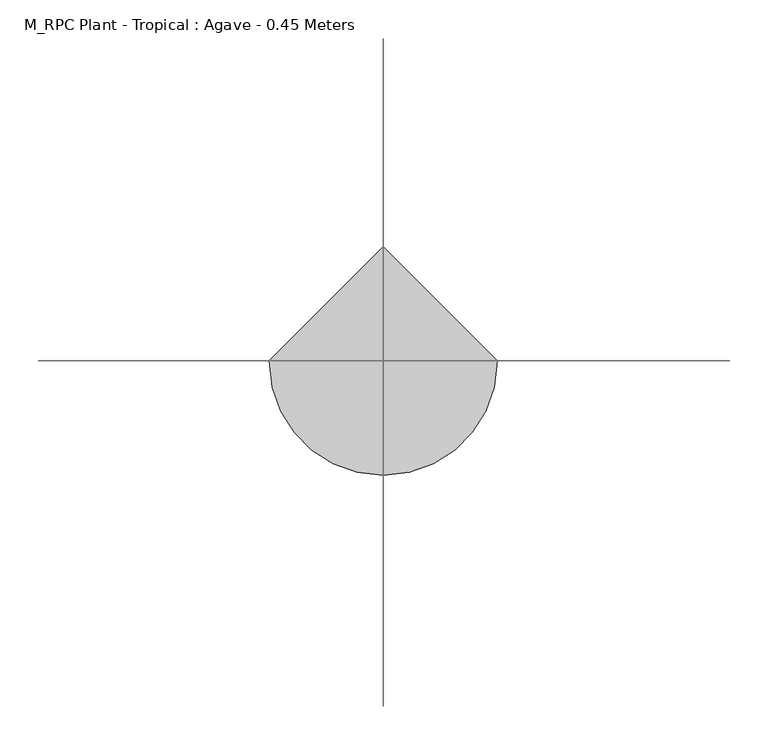
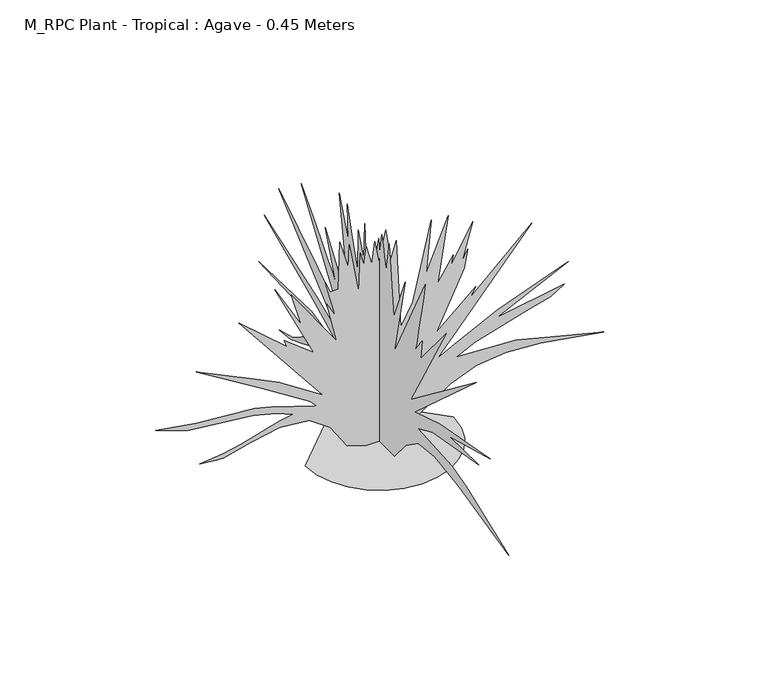
"""IFC4 building model written with IfcOpenShell, lengths in millimetres: geographic element geometry, M_RPC Plant - Tropical : Agave - 0.45 Meters."""

from ifc_helpers import new_model, si_unit, origin, place, context, project, spatial, triangles, source, transform, mapped, element, save


def m_rpc_plant_tropical_agave_0_45_meters_1685f993(model_context):
    return source(origin(), model_context, "Body", "Tessellation", [
        triangles([(-148.1386958, 0.0, 9.3e-06), (-144.2171964, -33.9885277, 9.3e-06), (-133.048683, -65.2018023, 9.3e-06), (-115.5276685, -92.7450748, 9.3e-06), (-92.5484025, -115.7243407, 9.3e-06), (-65.0051301, -133.2453552, 9.3e-06), (-33.7918577, -144.4138686, 9.3e-06), (0.1966776, -148.335368, 9.3e-06), (34.1851976, -144.4138686, 9.3e-06), (65.3984745, -133.2453552, 9.3e-06), (92.941747, -115.7243407, 9.3e-06), (115.921013, -92.7450748, 9.3e-06), (133.4420274, -65.2018023, 9.3e-06), (144.6105409, -33.9885277, 9.3e-06), (148.5320402, 1.3e-05, 9.3e-06), (0.1966516, 148.335368, 9.3e-06), (-24.3504259, 1.1e-06, 2.5e-06), (-64.1988793, 2e-06, 12.9348607), (-97.895905, 5e-07, 64.0713026), (-140.594189, 5e-07, 94.1593235), (-198.9417449, 2.8e-06, 99.5475847), (-255.4485429, 5.9e-06, 87.7748204), (-311.5910826, 9.2e-06, 73.8080584), (-324.2335885, 9.8e-06, 74.3145591), (-359.378609, 1.11e-05, 77.950311), (-313.1035629, 8.8e-06, 82.7858171), (-277.6960585, 6.8e-06, 90.344322), (-199.7057426, 2e-06, 113.0485956), (-172.7469775, 5e-07, 117.942592), (-204.8844963, 1.2e-06, 130.9928583), (-252.5285358, 2.5e-06, 143.4918682), (-382.9561306, 7.4e-06, 157.5558808), (-447.8461741, 8.9e-06, 179.7488939), (-367.8611217, 6.2e-06, 166.4181305), (-249.0960418, 1.6e-06, 156.7231191), (-216.6905162, 6e-07, 148.7013704), (-125.4831837, -1.6e-06, 119.1546001), (-138.0646922, -1.9e-06, 133.1736118), (-234.3990283, -1.3e-06, 193.9569111), (-366.6486231, -4e-07, 275.4877267), (-252.1085396, -2.1e-06, 220.5199336), (-200.6204942, -2.9e-06, 195.5036553), (-113.3644194, -3.3e-06, 138.5448591), (-281.816065, -8.5e-06, 349.4127929), (-184.8657327, -7.8e-06, 265.7927153), (-189.7134928, -8.4e-06, 280.3352324), (-131.5426884, -8.2e-06, 234.2839372), (-209.1037518, -1.44e-05, 395.4653234), (-155.7804623, -1.12e-05, 302.1502526), (-176.3827294, -1.45e-05, 372.4403117), (-85.4908937, -1.07e-05, 242.7671948), (-104.8811618, -1.49e-05, 327.6002798), (-87.9146465, -1.39e-05, 297.3027469), (-108.5169137, -1.76e-05, 374.8628019), (-97.9506527, -1.66e-05, 351.3077717), (-81.76514, -1.74e-05, 351.3277923), (-79.4313889, -2.33e-05, 450.0003668), (-62.2313804, -2.06e-05, 390.7203006), (-60.0411253, -2.35e-05, 437.880358), (-40.6511115, -1.79e-05, 330.02277), (-38.2271089, -2.29e-05, 412.4328197), (-30.9558549, -2.16e-05, 384.5578134), (-26.1083514, -2.4e-05, 422.1278312), (-15.2013409, -2.2e-05, 380.9228245), (-9.1419117, -2.5e-05, 426.9753551), (-0.6586671, -2.27e-05, 380.9228245), (12.6721065, -2.7e-05, 443.9403442), (23.5791135, -2.35e-05, 377.2877993), (34.4861967, -2.62e-05, 413.6428476), (42.9694566, -1.54e-05, 227.0126877), (67.2069761, -1.91e-05, 271.8527196), (104.0335027, -3.03e-05, 433.0253491), (93.8687435, -2.34e-05, 323.9627475), (138.4672839, -3.17e-05, 430.0728404), (116.8945182, -2.27e-05, 294.8777314), (148.4037959, -2.69e-05, 343.3552774), (143.5562902, -2.54e-05, 321.5402573), (187.184323, -3.2e-05, 400.312811), (165.3703021, -2.65e-05, 322.7527559), (177.4890573, -2.84e-05, 345.7777677), (170.9330439, -2.58e-05, 308.0802504), (114.4707654, -1.64e-05, 190.6558953), (193.2438187, -2.4e-05, 260.9452096), (181.1248092, -2.22e-05, 240.3434511), (305.9494211, -3.46e-05, 355.4727791), (116.8945182, -1.32e-05, 136.120861), (156.175787, -1.61e-05, 155.588123), (236.8716063, -2.2e-05, 195.5036553), (378.6619886, -3.14e-05, 248.8267087), (235.6598525, -2.1e-05, 179.7488939), (371.0494809, -2.83e-05, 203.1156725), (343.871961, -2.62e-05, 186.8916447), (295.8769073, -2.33e-05, 173.2968894), (192.5770716, -1.7e-05, 143.7823665), (154.4632825, -1.42e-05, 125.2138505), (274.4393895, -1.91e-05, 119.1546001), (331.2944584, -2.07e-05, 104.4295814), (450.1645283, -2.41e-05, 74.3145591), (324.0894476, -1.98e-05, 94.6895782), (253.5743659, -1.7e-05, 99.5105775), (194.5445751, -1.4e-05, 92.6238249), (142.6707883, -1.05e-05, 72.2130568), (85.3409936, -5.7e-06, 33.5950265), (32.7349455, -1.4e-06, 0.0), (0.196672, 19.7673413, 8.9e-06), (0.1966732, 47.0472873, 9.8e-06), (0.1966747, 67.3315551, 19.7666418), (0.1966772, 98.1250789, 58.1885449), (0.1966793, 130.6278551, 79.4465678), (0.1966812, 171.5303912, 83.5105639), (0.1966824, 205.2991693, 71.7218077), (0.1966844, 267.9552104, 45.114788), (0.1966857, 307.0702466, 29.8075238), (0.1966874, 347.7627846, 24.6271691), (0.1966857, 300.5702436, 38.2485329), (0.1966843, 245.8184439, 73.6468083), (0.1966827, 196.7091595, 96.1225757), (0.196681, 158.7086266, 94.9168263), (0.1966826, 185.5584048, 108.6283349), (0.1966859, 252.0827055, 120.1018443), (0.1966936, 419.0128324, 127.5108488), (0.1966855, 235.0574365, 132.4853544), (0.1966818, 162.3476305, 116.8738436), (0.1966792, 117.5043466, 94.9168263), (0.1966819, 157.4268734, 125.6566015), (0.1966862, 230.1374425, 162.6691225), (0.196696, 399.8753377, 236.7079353), (0.1966859, 214.4554237, 174.9013882), (0.1966819, 145.377618, 145.8161177), (0.1966963, 348.9752832, 323.9627475), (0.1966833, 143.900864, 195.427915), (0.1966945, 270.2027113, 382.1353231), (0.1966926, 244.8639419, 353.83527), (0.1966907, 220.4639232, 326.4102725), (0.1966889, 197.940407, 300.737748), (0.1966873, 178.2316355, 277.6927156), (0.196686, 162.2761232, 258.1477059), (0.1966851, 151.0121214, 242.9834425), (0.1966845, 145.377618, 233.0721834), (0.1966896, 187.793897, 339.7177814), (0.196686, 146.5683701, 279.2777206), (0.1966856, 142.6428648, 273.9577147), (0.1966852, 137.8938633, 268.4452241), (0.1966848, 132.4583575, 262.7727143), (0.1966844, 126.4736029, 256.975212), (0.1966839, 120.0768458, 251.0802049), (0.1966835, 113.405596, 245.1219566), (0.196683, 106.5973361, 239.1316973), (0.1966904, 138.1063594, 442.7278456), (0.1966867, 107.8090899, 361.5328016), (0.196689, 111.4448418, 435.4578678), (0.196687, 96.9023247, 386.9828107), (0.1966838, 73.8763092, 315.4802711), (0.1966864, 72.6643101, 403.9478362), (0.196684, 54.4860456, 353.0502889), (0.1966862, 50.8502891, 430.6103439), (0.1966844, 46.5152885, 378.1328058), (0.1966819, 26.6125221, 322.7527559), (0.1966839, 1.1628534, 429.3978453), (0.1966829, -1.2609561, 399.1003123), (0.1966839, -8.4154066, 443.3628722), (0.1966833, -11.789735, 429.27536), (0.1966828, -15.0040374, 415.6178361), (0.1966823, -17.8983397, 402.817818), (0.1966818, -20.312591, 391.3078011), (0.1966815, -22.0867923, 381.5153028), (0.1966812, -23.0609175, 373.8703116), (0.196681, -23.0749678, 368.8028157), (0.1966826, -33.9820282, 439.0928567), (0.1966776, -49.7365399, 293.6677398), (0.1966787, -90.9408244, 393.0428332), (0.1966754, -52.1602928, 222.165182), (0.1966767, -160.0183758, 429.3978453), (0.1966761, -153.4961177, 397.6378289), (0.1966754, -147.1613663, 367.0353001), (0.1966749, -141.2021097, 338.7452754), (0.1966744, -135.8058639, 313.9252424), (0.196674, -131.1606078, 293.7327431), (0.1966737, -127.4541026, 279.3227215), (0.1966736, -124.8736006, 271.8527196), (0.1966736, -124.0245972, 269.8952265), (0.1966736, -125.1655977, 270.9177113), (0.1966735, -127.9646002, 274.4252189), (0.1966735, -132.090611, 279.9202323), (0.1966735, -137.211365, 286.9052347), (0.1966735, -142.995614, 294.8852345), (0.1966734, -149.1113744, 303.3627512), (0.1966725, -143.0521149, 262.1577082), (0.1966717, -232.7319426, 370.0153144), (0.1966708, -109.1190844, 155.5111291), (0.1966659, -335.7427697, 328.8102714), (0.1966697, -122.4498477, 136.1211063), (0.1966666, -209.7059134, 163.9943868), (0.1966597, -385.1278004, 196.2989011), (0.196665, -242.426954, 157.9348729), (0.1966604, -345.9302656, 160.358871), (0.1966667, -186.3451482, 131.3988564), (0.1966683, -133.3568582, 108.2475896), (0.1966628, -253.3352089, 100.9760858), (0.1966602, -301.8102479, 87.6453225), (0.1966519, -448.4478453, 30.686524), (0.196661, -273.6277203, 71.7218077), (0.196665, -192.0614054, 83.6695659), (0.1966673, -135.4426139, 77.7298121), (0.1966684, -92.7000739, 48.0972868), (0.1966688, -51.7737929, 6.8e-06), (0.1966702, -18.8243404, 7.8e-06)], [[15, 16, 1], [14, 15, 1], [14, 1, 2], [13, 14, 2], [13, 2, 3], [13, 3, 4], [12, 13, 4], [11, 12, 4], [11, 4, 5], [11, 5, 6], [11, 6, 7], [11, 7, 8], [11, 8, 9], [11, 9, 10], [47, 48, 49], [97, 98, 99], [88, 89, 90], [39, 40, 41], [84, 85, 86], [71, 72, 73], [53, 54, 55], [32, 33, 34], [43, 44, 45], [24, 25, 26], [58, 59, 60], [77, 78, 79], [73, 74, 75], [60, 61, 62], [51, 52, 53], [56, 57, 58], [82, 83, 84], [79, 80, 81], [64, 65, 66], [49, 50, 51], [68, 69, 70], [75, 76, 77], [90, 91, 92], [90, 92, 93], [66, 67, 68], [82, 84, 86], [90, 93, 94], [62, 63, 64], [47, 49, 51], [39, 41, 42], [45, 46, 47], [43, 45, 47], [38, 39, 42], [38, 42, 43], [31, 32, 34], [31, 34, 35], [23, 24, 26], [56, 58, 60], [87, 88, 90], [87, 90, 94], [87, 94, 95], [37, 38, 43], [86, 87, 95], [71, 73, 75], [96, 97, 99], [96, 99, 100], [95, 96, 100], [95, 100, 101], [95, 101, 102], [53, 55, 56], [53, 56, 60], [22, 23, 26], [22, 26, 27], [22, 27, 28], [21, 22, 28], [60, 62, 64], [43, 47, 51], [30, 31, 35], [30, 35, 36], [30, 36, 37], [29, 30, 37], [86, 95, 102], [21, 28, 29], [20, 21, 29], [20, 29, 37], [19, 20, 37], [86, 102, 103], [66, 68, 70], [64, 66, 70], [60, 64, 70], [53, 60, 70], [51, 53, 70], [43, 51, 70], [77, 79, 81], [77, 81, 82], [75, 77, 82], [71, 75, 82], [70, 71, 82], [70, 82, 86], [43, 70, 86], [43, 86, 103], [43, 103, 104], [43, 104, 17], [43, 17, 18], [43, 18, 19], [43, 19, 37], [120, 121, 122], [193, 194, 195], [190, 191, 192], [126, 127, 128], [155, 156, 157], [131, 132, 133], [200, 201, 202], [113, 114, 115], [195, 196, 197], [129, 130, 131], [131, 133, 134], [170, 171, 172], [188, 189, 190], [131, 134, 135], [148, 149, 150], [139, 140, 141], [131, 135, 136], [150, 151, 152], [168, 169, 170], [172, 173, 174], [131, 136, 137], [158, 159, 160], [172, 174, 175], [131, 137, 138], [153, 154, 155], [131, 138, 139], [172, 175, 176], [160, 161, 162], [172, 176, 177], [186, 187, 188], [172, 177, 178], [112, 113, 115], [112, 115, 116], [111, 112, 116], [111, 116, 117], [160, 162, 163], [172, 178, 179], [172, 179, 180], [172, 180, 181], [139, 141, 142], [193, 195, 197], [185, 186, 188], [192, 193, 197], [192, 197, 198], [155, 157, 158], [150, 152, 153], [148, 150, 153], [139, 142, 143], [199, 200, 202], [119, 120, 122], [119, 122, 123], [118, 119, 123], [199, 202, 203], [198, 199, 203], [198, 203, 204], [184, 185, 188], [110, 111, 117], [110, 117, 118], [109, 110, 118], [160, 163, 164], [118, 123, 124], [109, 118, 124], [139, 143, 144], [125, 126, 128], [125, 128, 129], [183, 184, 188], [139, 144, 145], [153, 155, 158], [108, 109, 124], [139, 145, 146], [160, 164, 165], [158, 160, 165], [158, 165, 166], [158, 166, 167], [158, 167, 168], [158, 168, 170], [182, 183, 188], [124, 125, 129], [182, 188, 190], [181, 182, 190], [172, 181, 190], [139, 146, 147], [131, 139, 147], [131, 147, 148], [158, 170, 172], [153, 158, 172], [148, 153, 172], [198, 204, 205], [131, 148, 172], [129, 131, 172], [124, 129, 172], [124, 172, 190], [108, 124, 190], [107, 108, 190], [106, 107, 190], [105, 106, 190], [207, 105, 190], [206, 207, 190], [205, 206, 190], [198, 205, 190], [192, 198, 190]], closed=False),
    ])


if __name__ == "__main__":
    model = new_model("IFC4")
    model_context = context("Model", 3, world=origin())
    ifc_project = project(units=[si_unit("LENGTHUNIT", "METRE", prefix="MILLI")], contexts=[model_context])
    site = spatial("IfcSite", under=ifc_project)
    building = spatial("IfcBuilding", under=site)
    placement = place(None, origin())
    m_rpc_plant_tropical_agave_0_45_meters_shape = m_rpc_plant_tropical_agave_0_45_meters_1685f993(model_context)
    element("IfcGeographicElement", 1, ObjectType="M_RPC Plant - Tropical : Agave - 0.45 Meters", at=placement, inside=building, context=model_context, shape_type="MappedRepresentation", body=[
        mapped(m_rpc_plant_tropical_agave_0_45_meters_shape, transform((0.0, 0.0, 0.0), x_axis=(1.0, 0.0, 0.0), y_axis=(0.0, 1.0, 0.0), z_axis=(0.0, 0.0, 1.0))),
    ])
    save(model, "model.ifc")

# Revit data of these elements
# Type "M_RPC Plant - Tropical : Agave - 0.45 Meters"
#   built-in parameter 1005198 = "{2, 15},{39, RPC-16-G1GJ-63FX-7K5P-N000-ST1L-LVER-AU},{1, 0},{1, 0},{2, 35},{1, 8},{5, Color},{1, 0},{1, 0},{3, 0.8},{3, 0.8},{3, 0.8},{1, 8},{7, BBoxMin},{1, 0},{1, 0},{1, 0},{1, 0},{1, 0},{1, 8},{7, BBoxMax},{1, 0},{1, 0},{1, 0},{1, 0},{1, 0},{2, 11},{9, RPCTypeId},{1, 0},{1, 0},{39, RPC-16-G1GJ-63FX-7K5P-N000-ST1L-LVER-AU},{1, 6},{14, RPCPlantHeight},{1, 0},{1, 0},{7, 1.47638},{2, 11},{7, keyword},{1, 0},{1, 0},{88, :Geometry:RPC:Agave:agave:agave americana marginata:mesqual:south western:tropical:plant},{2, 11},{8, category},{1, 0},{1, 0},{17, :Plants [General]},{2, 11},{12, LocalizedUID},{1, 0},{1, 0},{5, Agave},{2, 14},{6, Height},{1, 0},{1, 0},{7, 1.47638},{1, 2},{16, Cast Reflections},{1, 0},{1, 0},{1, 0},{1, 2},{12, Cast Shadows},{1, 0},{1, 0},{1, 1},{1, 2},{9, Lock View},{1, 0},{1, 0},{1, 0},{1, 4},{5, ViewC},{1, 0},{1, 0},{1, 0},{2, 11},{20, AdvancedUIDefinition},{1, 0},{1, 0},{0, },{2, 11},{10, AssetLibID},{1, 0},{1, 0},{36, 4D3F6E72-3F99-4203-98E9-AF80B3C7A7A4},{2, 11},{10, BaseSchema},{1, 0},{1, 0},{9, RPCSchema},{2, 11},{12, ExchangeGUID},{1, 0},{1, 0},{0, },{1, 2},{6, Hidden},{1, 0},{1, 0},{1, 0},{1, 4},{11, RPCCategory},{1, 0},{1, 0},{1, 0},{2, 11},{8, RPCImage},{1, 0},{1, 0},{0, },{1, 4},{13, SchemaVersion},{1, 0},{1, 0},{1, 4},{2, 11},{12, UIDefinition},{1, 0},{1, 0},{0, },{2, 11},{6, UIName},{1, 0},{1, 0},{39, RPC-16-G1GJ-63FX-7K5P-N000-ST1L-LVER-AU},{2, 11},{11, VersionGUID},{1, 0},{1, 0},{9, RPCSchema},{2, 11},{9, assettype},{1, 0},{1, 0},{11, RPCGeometry},{2, 11},{11, description},{1, 0},{1, 0},{0, },{2, 11},{9, localname},{1, 0},{1, 0},{3, RPC},{2, 11},{9, localtype},{1, 0},{1, 0},{3, RPC},{1, 4},{8, revision},{1, 0},{1, 0},{1, 1},{2, 11},{9, thumbnail},{1, 0},{1, 0},{0, },{1, 4},{7, version},{1, 0},{1, 0},{1, 1},{1, 2},{20, RPC_Cast Reflections},{1, 0},{1, 0},{1, 1},{1, 2},{16, RPC_Cast Shadows},{1, 0},{1, 0},{1, 1},{1, 2},{13, RPC_Lock View},{1, 0},{1, 0},{1, 0},{1, 4},{9, RPC_ViewC},{1, 0},{1, 0},{1, 0},{21, assetlibrary_base.fbx},{1, 5},"
#   built-in parameter 1005195 = "RPC-16-G1GJ-63FX-7K5P-N000-ST1L-LVER-AU"
#   Type Comments = "Agave"
#   Height = 0.45 m
#   Description = (empty or 0)
#   Default Elevation = 0
